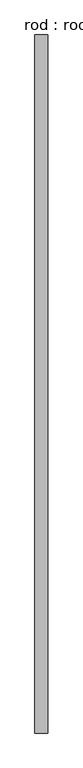
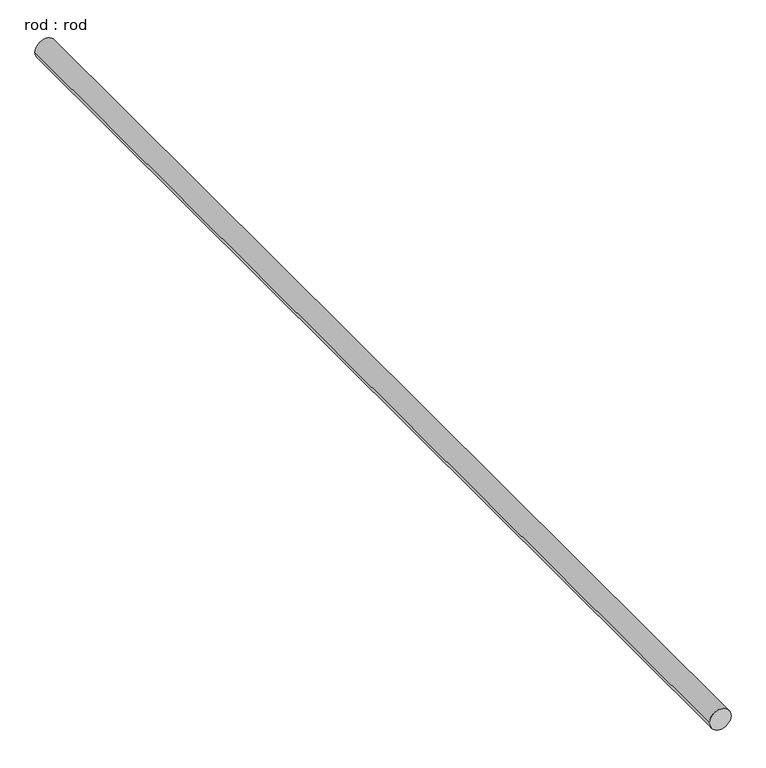
"""IFC4 building model written with IfcOpenShell, lengths in millimetres: proxy geometry, rod : rod."""

from ifc_helpers import new_model, si_unit, point, frame, frame_2d, origin, place, context, project, spatial, circle_curve, trimmed, segment, composite_curve, outline, extrude, source, transform, mapped, element, save


def rod_rod_ca47f08f(model_context):
    return source(origin(), model_context, "Body", "SweptSolid", [
        extrude(outline(composite_curve([segment(trimmed(circle_curve(frame_2d((0.0108462, 0.0)), 200.0), [point((0.0108462, 200.0))], [point((0.0108462, -200.0))], False, "CARTESIAN"), True, "CONTINUOUS"), segment(trimmed(circle_curve(frame_2d((0.0108462, 0.0)), 200.0), [point((0.0108462, -200.0))], [point((0.0108462, 200.0))], False, "CARTESIAN"), True, "CONTINUOUS")], self_intersect=False)), frame((0.0, -6699.1305946, 0.0), z_axis=(0.0, 1.0, 0.0), x_axis=(0.0, 0.0, 1.0)), (0.0, 0.0, 1.0), 21583.7184198),
    ])


if __name__ == "__main__":
    model = new_model("IFC4")
    model_context = context("Model", 3, world=origin())
    ifc_project = project(units=[si_unit("LENGTHUNIT", "METRE", prefix="MILLI")], contexts=[model_context])
    site = spatial("IfcSite", under=ifc_project)
    building = spatial("IfcBuilding", under=site)
    placement = place(None, origin())
    rod_rod_shape = rod_rod_ca47f08f(model_context)
    element("IfcBuildingElementProxy", 1, Name="rod : rod", ObjectType="rod : rod", at=placement, inside=building, context=model_context, shape_type="MappedRepresentation", body=[
        mapped(rod_rod_shape, transform((0.0, 0.0, 0.0), x_axis=(1.0, 0.0, 0.0), y_axis=(0.0, 1.0, 0.0), z_axis=(0.0, 0.0, 1.0))),
    ])
    save(model, "model.ifc")

# Revit data of these elements
# Type "rod : rod"
#   Default Elevation = 0
